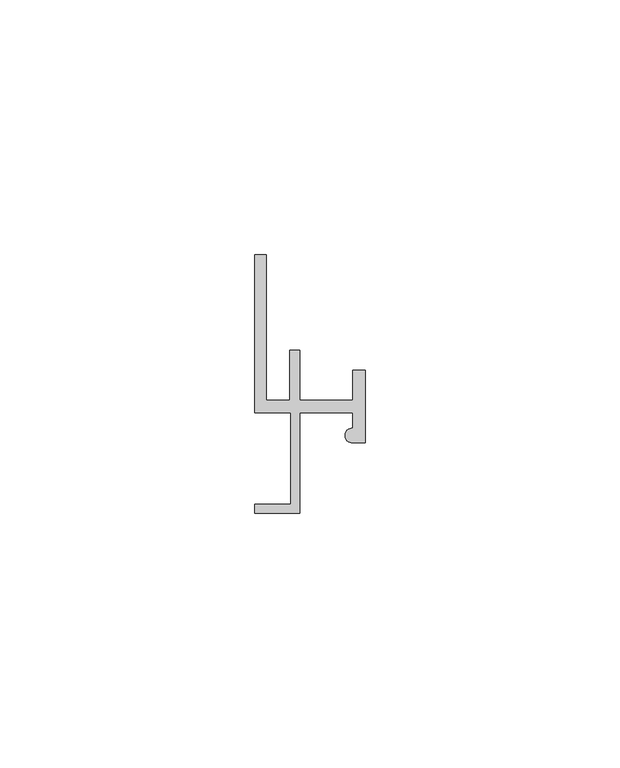
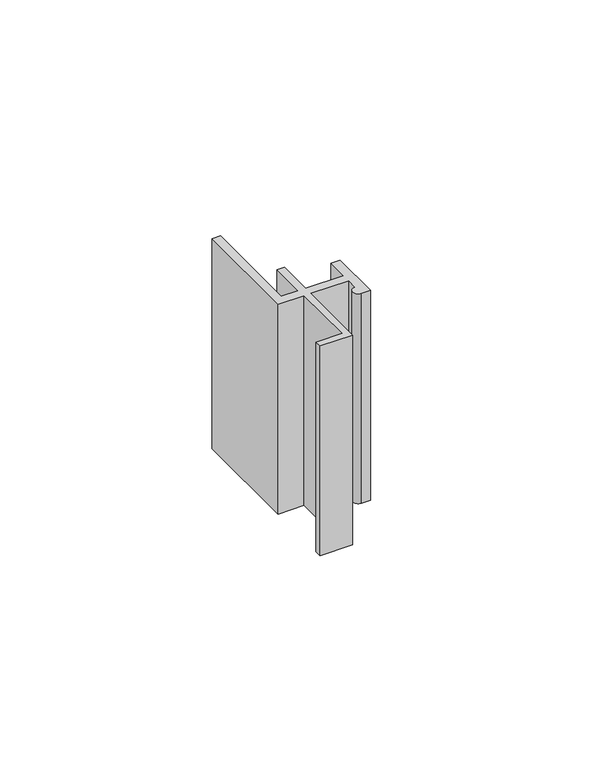
"""IFC4 building model written with IfcOpenShell, lengths in millimetres: proxy geometry, Generic Models 9:Generic Models 5:348123:Generic Models 5:348123 : Generic Models 9:Generic Models 5:348123:10 : Generic Models 9:Generic Models 5:348123:Generic Models 5:348123 : Generic Models 9:Generic Models 5:348123:301771."""

from ifc_helpers import new_model, si_unit, point, frame, frame_2d, origin, place, context, project, spatial, polyline, circle_curve, trimmed, segment, composite_curve, outline, extrude, source, transform, mapped, element, save


def generic_models_f78c31f2(model_context):
    return source(origin(), model_context, "Body", "SweptSolid", [
        extrude(outline(composite_curve([segment(polyline([(667556.1893938, -567733.9035817), (667556.1893938, -567753.631737), (667547.3117239, -567753.631737), (667547.3117239, -567751.856203), (667554.4138598, -567751.856203), (667554.4138598, -567733.9035817), (667547.3117239, -567733.9035817), (667547.3117239, -567702.831737), (667549.5804618, -567702.831737), (667549.5804618, -567731.4375622), (667554.2165783, -567731.4375622), (667554.2165783, -567721.5734846), (667556.1893938, -567721.5734846), (667556.1893938, -567731.4375622), (667566.5466754, -567731.4375622), (667566.5466754, -567725.5191156), (667569.0126948, -567725.5191156), (667569.0126948, -567739.8220283), (667566.5466754, -567739.8220283)]), True, "CONTINUOUS"), segment(trimmed(circle_curve(frame_2d((667566.5466754, -567738.3424166)), 1.4796117), [point((667566.5466754, -567739.8220283))], [point((667566.5466754, -567736.862805))], False, "CARTESIAN"), True, "CONTINUOUS"), segment(polyline([(667566.5466754, -567736.862805), (667566.5466754, -567733.9035817), (667556.1893938, -567733.9035817)]), True, "CONTINUOUS")], self_intersect=False)), frame((0.0, 0.0, 1315.803648), z_axis=(0.0, 0.0, 1.0), x_axis=(1.0, 0.0, 0.0)), (0.0, 0.0, 1.0), 60.325),
    ])


if __name__ == "__main__":
    model = new_model("IFC4")
    model_context = context("Model", 3, world=origin())
    ifc_project = project(units=[si_unit("LENGTHUNIT", "METRE", prefix="MILLI")], contexts=[model_context])
    site = spatial("IfcSite", under=ifc_project)
    building = spatial("IfcBuilding", under=site)
    placement = place(None, origin())
    generic_models_shape = generic_models_f78c31f2(model_context)
    element("IfcBuildingElementProxy", 1, Name="Generic Models 9:Generic Models 5:348123:Generic Models 5:348123 : Generic Models 9:Generic Models 5:348123:10 : Generic Models 9:Generic Models 5:348123:Generic Models 5:348123 : Generic Models 9:Generic Models 5:348123:301771", ObjectType="Generic Models 9:Generic Models 5:348123:Generic Models 5:348123 : Generic Models 9:Generic Models 5:348123:10 : Generic Models 9:Generic Models 5:348123:Generic Models 5:348123 : Generic Models 9:Generic Models 5:348123:301771", at=placement, inside=building, context=model_context, shape_type="MappedRepresentation", body=[
        mapped(generic_models_shape, transform((0.0, 0.0, 0.0), x_axis=(1.0, 0.0, 0.0), y_axis=(0.0, 1.0, 0.0), z_axis=(0.0, 0.0, 1.0))),
    ])
    save(model, "model.ifc")

# Revit data of these elements
# Type "Generic Models 9:Generic Models 5:348123:Generic Models 5:348123 : Generic Models 9:Generic Models 5:348123:10 : Generic Models 9:Generic Models 5:348123:Generic Models 5:348123 : Generic Models 9:Generic Models 5:348123:301771"
#   NameOverride = "Generic Models 9:Generic Models 5:348123:Generic Models 5:348123 : Generic Models 9:Generic Models 5:348123:301771"
#   ObjectTypeOverride = "Generic Models 5:348123 : Generic Models 9:Generic Models 5:348123"
#   Reference = "Generic Models 5"
#   Tag = "301771"
# Element 1 (IfcBuildingElementProxy, "Generic Models 9:Generic Models 5:348123:Generic Models 5:348123 : Generic Models 9:Generic Models 5:348123:10 : Generic Models 9:Generic Models 5:348123:Generic Models 5:348123 : Generic Models 9:Generic Models 5:348123:301771")
#   Materials on its faces: "GALVANIZED STEEL CLIP AT EVERY SEAM IN POLYCARBONATE"
# Materials
#   "GALVANIZED STEEL CLIP AT EVERY SEAM IN POLYCARBONATE": class "Unassigned", colour RGB 120 120 120, transparency 0, Cost = 0
